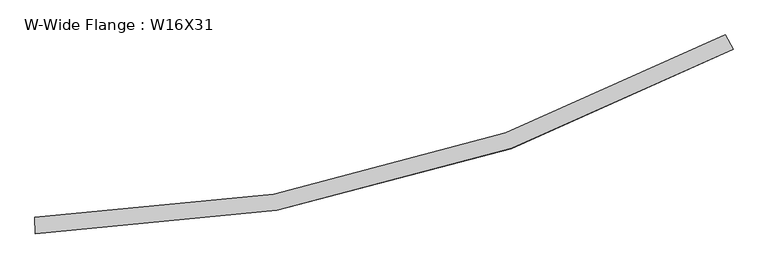
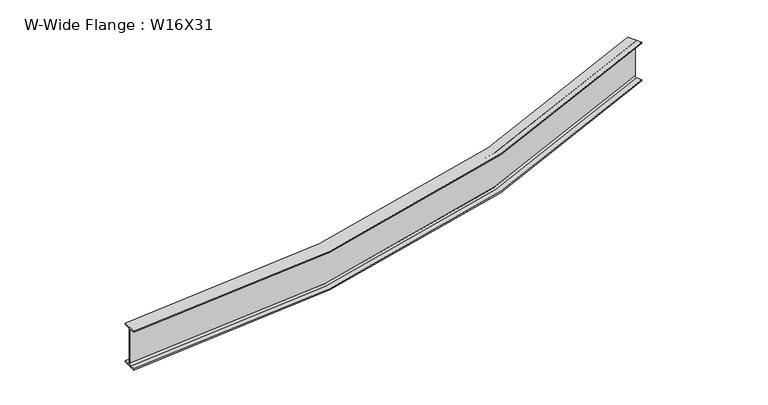
"""IFC4 building model written with IfcOpenShell, lengths in millimetres: beam geometry, W-Wide Flange : W16X31."""

from ifc_helpers import new_model, si_unit, point, frame, origin, place, context, project, spatial, polyline, circle_curve, ellipse_curve, trimmed, source, transform, mapped, element, save
from ifc_brep_helpers import plane_surface, cylinder_surface, revolved_surface, advanced_brep


def w_wide_flange_w16x31_8ecb8886(model_context):
    return source(origin(), model_context, "Body", "AdvancedBrep", [
        advanced_brep(
        [(6106.6437094, 1493.8987471, -190.754), (6106.6437094, 1493.8987471, -201.93), (6039.1190231, 1617.0652612, -201.93), (6039.1190231, 1617.0652612, -190.754), (6062.8381376, 1573.8010743, -190.754), (6071.202407, 1558.5444627, -173.355), (6071.202407, 1558.5444627, 173.355), (6062.8381376, 1573.8010743, 190.754), (6039.1190231, 1617.0652612, 190.754), (6039.1190231, 1617.0652612, 201.93), (6106.6437094, 1493.8987471, 201.93), (6106.6437094, 1493.8987471, 190.754), (6082.9245949, 1537.162934, 190.754), (6074.5603254, 1552.4195456, 173.355), (6074.5603254, 1552.4195456, -173.355), (6082.9245949, 1537.162934, -190.754), (187.278858, -68.8503861, -190.754), (186.551439, -19.5162486, -190.754), (186.2949232, -2.1191396, -173.355), (186.2949232, -2.1191396, 173.355), (186.551439, -19.5162486, 190.754), (187.278858, -68.8503861, 190.754), (187.278858, -68.8503861, 201.93), (185.2080076, 71.5963477, 201.93), (185.2080076, 71.5963477, 190.754), (185.9354266, 22.2622102, 190.754), (186.1919424, 4.8651012, 173.355), (186.1919424, 4.8651012, -173.355), (185.9354266, 22.2622102, -190.754), (185.2080076, 71.5963477, -190.754), (185.2080076, 71.5963477, -201.93), (187.278858, -68.8503861, -201.93)],
        [
            (0, 1),
            (1, 2),
            (2, 3),
            (3, 4),
            (4, 5, circle_curve(frame((6062.8381376, 1573.8010743, -173.355), z_axis=(-0.8768671529491879, -0.48073276992398356, 0.0), x_axis=(-0.48073276992398356, 0.8768671529491879, 0.0)), 17.399)),
            (5, 6),
            (6, 7, circle_curve(frame((6062.8381376, 1573.8010743, 173.355), z_axis=(-0.8768671529491879, -0.48073276992398356, 0.0), x_axis=(-0.48073276992398356, 0.8768671529491879, 0.0)), 17.399)),
            (7, 8),
            (8, 9),
            (9, 10),
            (10, 11),
            (11, 12),
            (12, 13, circle_curve(frame((6082.9245949, 1537.162934, 173.355), z_axis=(-0.8768671529491879, -0.48073276992398356, 0.0), x_axis=(-0.48073276992398356, 0.8768671529491879, 0.0)), 17.399)),
            (13, 14),
            (14, 15, circle_curve(frame((6082.9245949, 1537.162934, -173.355), z_axis=(-0.8768671529491879, -0.48073276992398356, 0.0), x_axis=(-0.48073276992398356, 0.8768671529491879, 0.0)), 17.399)),
            (15, 0),
            (16, 17),
            (17, 18, circle_curve(frame((186.551439, -19.5162486, -173.355), z_axis=(0.999891314050926, 0.014743136895264575, 0.0), x_axis=(-0.014743136895264575, 0.999891314050926, 0.0)), 17.399)),
            (18, 19),
            (19, 20, circle_curve(frame((186.551439, -19.5162486, 173.355), z_axis=(0.999891314050926, 0.014743136895264575, 0.0), x_axis=(-0.014743136895264575, 0.999891314050926, 0.0)), 17.399)),
            (20, 21),
            (21, 22),
            (22, 23),
            (23, 24),
            (24, 25),
            (25, 26, circle_curve(frame((185.9354266, 22.2622102, 173.355), z_axis=(0.999891314050926, 0.014743136895264575, 0.0), x_axis=(-0.014743136895264575, 0.999891314050926, 0.0)), 17.399)),
            (26, 27),
            (27, 28, circle_curve(frame((185.9354266, 22.2622102, -173.355), z_axis=(0.999891314050926, 0.014743136895264575, 0.0), x_axis=(-0.014743136895264575, 0.999891314050926, 0.0)), 17.399)),
            (28, 29),
            (29, 30),
            (30, 31),
            (31, 16),
            (15, 17, circle_curve(frame((0.0, 12632.5512762, -190.754), z_axis=(0.0, 0.0, -1.0), x_axis=(-0.5014171979932397, 0.8652056365723748, 0.0)), 12653.4427762)),
            (16, 0, circle_curve(frame((0.0, 12632.5512762, -190.754), z_axis=(0.0, 0.0, 1.0), x_axis=(-0.5014171979932397, 0.8652056365723748, 0.0)), 12702.7822762)),
            (14, 18, circle_curve(frame((0.0, 12632.5512762, -173.355), z_axis=(0.0, 0.0, -1.0), x_axis=(-0.5014171979932397, 0.8652056365723748, 0.0)), 12636.0437762)),
            (13, 19, circle_curve(frame((0.0, 12632.5512762, 173.355), z_axis=(0.0, 0.0, -1.0), x_axis=(-0.5014171979932397, 0.8652056365723748, 0.0)), 12636.0437762)),
            (12, 20, circle_curve(frame((0.0, 12632.5512762, 190.754), z_axis=(0.0, 0.0, -1.0), x_axis=(-0.5014171979932397, 0.8652056365723748, 0.0)), 12653.4427762)),
            (11, 21, circle_curve(frame((0.0, 12632.5512762, 190.754), z_axis=(0.0, 0.0, -1.0), x_axis=(-0.5014171979932397, 0.8652056365723748, 0.0)), 12702.7822762)),
            (10, 22, circle_curve(frame((0.0, 12632.5512762, 201.93), z_axis=(0.0, 0.0, -1.0), x_axis=(-0.5014171979932397, 0.8652056365723748, 0.0)), 12702.7822762)),
            (9, 23, circle_curve(frame((0.0, 12632.5512762, 201.93), z_axis=(0.0, 0.0, -1.0), x_axis=(-0.5014171979932397, 0.8652056365723748, 0.0)), 12562.3202762)),
            (8, 24, circle_curve(frame((0.0, 12632.5512762, 190.754), z_axis=(0.0, 0.0, -1.0), x_axis=(-0.5014171979932397, 0.8652056365723748, 0.0)), 12562.3202762)),
            (7, 25, circle_curve(frame((0.0, 12632.5512762, 190.754), z_axis=(0.0, 0.0, -1.0), x_axis=(-0.5014171979932397, 0.8652056365723748, 0.0)), 12611.6597762)),
            (6, 26, circle_curve(frame((0.0, 12632.5512762, 173.355), z_axis=(0.0, 0.0, -1.0), x_axis=(-0.5014171979932397, 0.8652056365723748, 0.0)), 12629.0587762)),
            (5, 27, circle_curve(frame((0.0, 12632.5512762, -173.355), z_axis=(0.0, 0.0, -1.0), x_axis=(-0.5014171979932397, 0.8652056365723748, 0.0)), 12629.0587762)),
            (4, 28, circle_curve(frame((0.0, 12632.5512762, -190.754), z_axis=(0.0, 0.0, -1.0), x_axis=(-0.5014171979932397, 0.8652056365723748, 0.0)), 12611.6597762)),
            (3, 29, circle_curve(frame((0.0, 12632.5512762, -190.754), z_axis=(0.0, 0.0, -1.0), x_axis=(-0.5014171979932397, 0.8652056365723748, 0.0)), 12562.3202762)),
            (2, 30, circle_curve(frame((0.0, 12632.5512762, -201.93), z_axis=(0.0, 0.0, -1.0), x_axis=(-0.5014171979932397, 0.8652056365723748, 0.0)), 12562.3202762)),
            (1, 31, circle_curve(frame((0.0, 12632.5512762, -201.93), z_axis=(0.0, 0.0, -1.0), x_axis=(-0.5014171979932397, 0.8652056365723748, 0.0)), 12702.7822762)),
        ],
        [
            plane_surface(frame((6072.8813662, 1555.4820042, 0.0), z_axis=(0.8768671529491846, 0.4807327699239896, 0.0), x_axis=(0.0, 0.0, 1.0))),
            plane_surface(frame((186.2434328, 1.3729808, 0.0), z_axis=(-0.9998913140509259, -0.014743136895271347, 0.0), x_axis=(0.0, 0.0, 1.0))),
            plane_surface(frame((0.0, 12632.5512762, -190.754), z_axis=(0.0, 0.0, 1.0), x_axis=(-0.5014171979932397, 0.8652056365723748, 0.0))),
            revolved_surface(trimmed(ellipse_curve(frame((-6344.6538218, 23580.3812883, -173.355), z_axis=(0.8652056365723783, 0.5014171979932338, 0.0), x_axis=(0.5014171979932338, -0.8652056365723783, 0.0)), 17.399, 17.399), [point((-6335.929664, 23565.3275754, -173.355))], [point((-6344.6538218, 23580.3812883, -190.754))], True, "CARTESIAN"), (0.0, 12632.5512762, 0.0), (0.0, 0.0, -1.0)),
            cylinder_surface(frame((0.0, 12632.5512762, 0.0), z_axis=(0.0, 0.0, -1.0), x_axis=(-0.5014171979932397, 0.8652056365723748, 0.0)), 12636.0437762),
            revolved_surface(trimmed(ellipse_curve(frame((-6344.6538218, 23580.3812883, 173.355), z_axis=(0.8652056365723783, 0.5014171979932338, 0.0), x_axis=(0.5014171979932338, -0.8652056365723783, 0.0)), 17.399, 17.399), [point((-6344.6538218, 23580.3812883, 190.754))], [point((-6335.929664, 23565.3275754, 173.355))], True, "CARTESIAN"), (0.0, 12632.5512762, 0.0), (0.0, 0.0, -1.0)),
            plane_surface(frame((0.0, 12632.5512762, 190.754), z_axis=(0.0, 0.0, -1.0), x_axis=(-0.5014171979932397, 0.8652056365723748, 0.0))),
            cylinder_surface(frame((0.0, 12632.5512762, 0.0), z_axis=(0.0, 0.0, -1.0), x_axis=(-0.5014171979932397, 0.8652056365723748, 0.0)), 12702.7822762),
            plane_surface(frame((0.0, 12632.5512762, 201.93), z_axis=(0.0, 0.0, 1.0), x_axis=(-0.5014171979932397, 0.8652056365723748, 0.0))),
            revolved_surface(polyline([(-6298.963433185865, 23501.54158759567, 190.754), (-6298.963433185865, 23501.54158759567, 201.93)]), (0.0, 12632.5512762, 0.0), (0.0, 0.0, -1.0)),
            revolved_surface(trimmed(ellipse_curve(frame((-6323.703107, 23544.2304011, 173.355), z_axis=(0.8652056365723783, 0.5014171979932338, 0.0), x_axis=(0.5014171979932338, -0.8652056365723783, 0.0)), 17.399, 17.399), [point((-6332.4272649, 23559.284114, 173.355))], [point((-6323.703107, 23544.2304011, 190.754))], True, "CARTESIAN"), (0.0, 12632.5512762, 0.0), (0.0, 0.0, -1.0)),
            revolved_surface(polyline([(-6332.427264854136, 23559.284113972055, -173.355), (-6332.427264854136, 23559.284113972055, 173.355)]), (0.0, 12632.5512762, 0.0), (0.0, 0.0, -1.0)),
            revolved_surface(trimmed(ellipse_curve(frame((-6323.703107, 23544.2304011, -173.355), z_axis=(0.8652056365723783, 0.5014171979932338, 0.0), x_axis=(0.5014171979932338, -0.8652056365723783, 0.0)), 17.399, 17.399), [point((-6323.703107, 23544.2304011, -190.754))], [point((-6332.4272649, 23559.284114, -173.355))], True, "CARTESIAN"), (0.0, 12632.5512762, 0.0), (0.0, 0.0, -1.0)),
            revolved_surface(polyline([(-6298.963433185865, 23501.54158759567, -201.93), (-6298.963433185865, 23501.54158759567, -190.754)]), (0.0, 12632.5512762, 0.0), (0.0, 0.0, -1.0)),
            plane_surface(frame((0.0, 12632.5512762, -201.93), z_axis=(0.0, 0.0, -1.0), x_axis=(-0.5014171979932397, 0.8652056365723748, 0.0))),
        ],
        [
            (0, [[1, 2, 3, 4, 5, 6, 7, 8, 9, 10, 11, 12, 13, 14, 15, 16]]),
            (1, [[17, 18, 19, 20, 21, 22, 23, 24, 25, 26, 27, 28, 29, 30, 31, 32]]),
            (2, [[33, -17, 34, -16]]),
            (3, [[35, -18, -33, -15]]),
            (4, [[36, -19, -35, -14]]),
            (5, [[37, -20, -36, -13]]),
            (6, [[38, -21, -37, -12]]),
            (7, [[39, -22, -38, -11]]),
            (8, [[40, -23, -39, -10]]),
            (9, [[41, -24, -40, -9]]),
            (6, [[42, -25, -41, -8]]),
            (10, [[43, -26, -42, -7]]),
            (11, [[44, -27, -43, -6]]),
            (12, [[45, -28, -44, -5]]),
            (2, [[46, -29, -45, -4]]),
            (13, [[47, -30, -46, -3]]),
            (14, [[48, -31, -47, -2]]),
            (7, [[-34, -32, -48, -1]]),
        ],
    ),
    ])


if __name__ == "__main__":
    model = new_model("IFC4")
    model_context = context("Model", 3, world=origin())
    ifc_project = project(units=[si_unit("LENGTHUNIT", "METRE", prefix="MILLI")], contexts=[model_context])
    site = spatial("IfcSite", under=ifc_project)
    building = spatial("IfcBuilding", under=site)
    placement = place(None, origin())
    w_wide_flange_w16x31_shape = w_wide_flange_w16x31_8ecb8886(model_context)
    element("IfcBeam", 1, ObjectType="W-Wide Flange : W16X31", at=placement, inside=building, context=model_context, shape_type="MappedRepresentation", body=[
        mapped(w_wide_flange_w16x31_shape, transform((0.0, 0.0, 0.0), x_axis=(1.0, 0.0, 0.0), y_axis=(0.0, 1.0, 0.0), z_axis=(0.0, 0.0, 1.0))),
    ])
    save(model, "model.ifc")

# Revit data of these elements
# Type "W-Wide Flange : W16X31"
#   Assembly Code = "B10"
#   W = 31
#   Start Extension Calculation [instance default] = 10' - 0"
#   Start Extension [instance default] = -0' - 0 1/2"
#   End Extension Calculation [instance default] = 10' - 0"
#   End Extension [instance default] = -0' - 0 1/2"
#   Length [instance default] = 5' - 0"
#   bf = 0' - 5.53"
#   d = 1' - 3.9"
#   k = 0' - 1 1/8"
#   k2 = 0' - 0.685"
#   tf = 0' - 0.44"
#   tw = 0' - 0.275"
#   A = 0.0634028 SF
#   Beam Material [instance default] = Metal - Steel - ASTM A992
# Element 1 (IfcBeam, "W-Wide Flange : W16X31")
#   Materials on its faces: "Metal - Steel - ASTM A992"
# Materials
#   "Metal - Steel - ASTM A992": class "Metal", colour RGB 128 0 0, transparency 0
